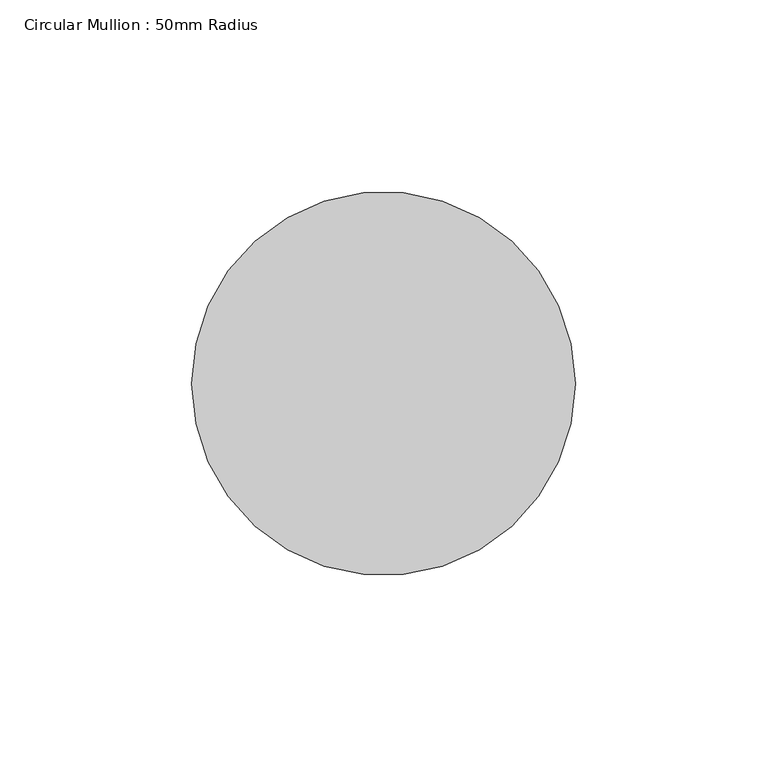
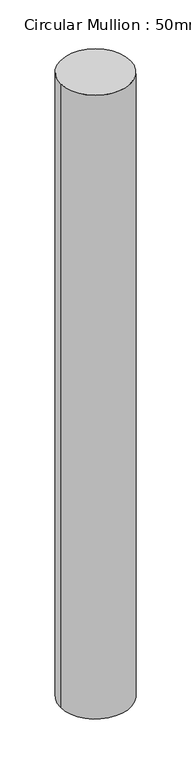
"""IFC4 building model written with IfcOpenShell, lengths in millimetres: member geometry, Circular Mullion : 50mm Radius."""

from ifc_helpers import new_model, si_unit, point, frame, origin, origin_2d, place, context, project, spatial, circle_curve, trimmed, segment, composite_curve, outline, extrude, source, transform, mapped, element, save


def circular_mullion_50mm_radius_5af3a7dd(model_context):
    return source(origin(), model_context, "Body", "SweptSolid", [
        extrude(outline(composite_curve([segment(trimmed(circle_curve(origin_2d(), 50.0), [point((50.0, 0.0))], [point((-50.0, 0.0))], False, "CARTESIAN"), True, "CONTINUOUS"), segment(trimmed(circle_curve(origin_2d(), 50.0), [point((-50.0, 0.0))], [point((50.0, 0.0))], False, "CARTESIAN"), True, "CONTINUOUS")], self_intersect=False)), frame((0.0, 0.0, -941.5935963), z_axis=(0.0, 0.0, 1.0), x_axis=(1.0, 0.0, 0.0)), (0.0, 0.0, 1.0), 941.5935963),
    ])


if __name__ == "__main__":
    model = new_model("IFC4")
    model_context = context("Model", 3, world=origin())
    ifc_project = project(units=[si_unit("LENGTHUNIT", "METRE", prefix="MILLI")], contexts=[model_context])
    site = spatial("IfcSite", under=ifc_project)
    building = spatial("IfcBuilding", under=site)
    placement = place(None, origin())
    circular_mullion_50mm_radius_shape = circular_mullion_50mm_radius_5af3a7dd(model_context)
    element("IfcMember", 1, ObjectType="Circular Mullion : 50mm Radius", at=placement, inside=building, context=model_context, shape_type="MappedRepresentation", body=[
        mapped(circular_mullion_50mm_radius_shape, transform((0.0, 0.0, 0.0), x_axis=(1.0, 0.0, 0.0), y_axis=(0.0, 1.0, 0.0), z_axis=(0.0, 0.0, 1.0))),
    ])
    save(model, "model.ifc")

# Revit data of these elements
# Type "Circular Mullion : 50mm Radius"
#   built-in parameter 1007350 = 0.164042 (stored number, unit not read)
# Element 1 (IfcMember, "Circular Mullion : 50mm Radius")
#   Materials on its faces: "Aluminium"
# Materials
#   "Aluminium": class "Metal", colour RGB 247 247 247, transparency 0, Description = "Aluminium 6061", Cost = 0
